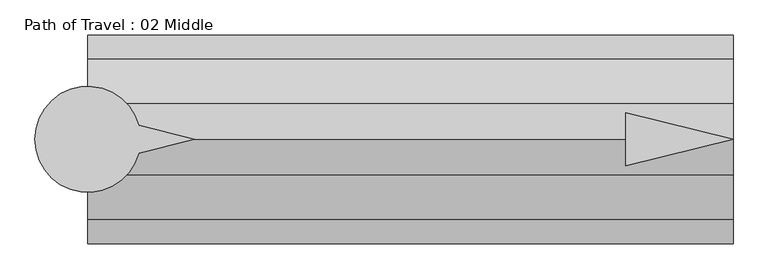
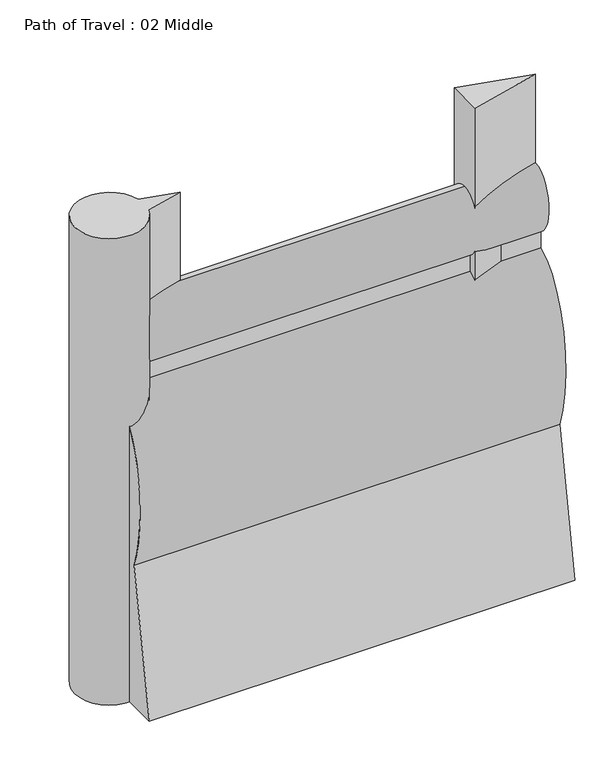
"""IFC4 building model written with IfcOpenShell, lengths in millimetres: proxy geometry, Path of Travel : 02 Middle."""

from ifc_helpers import new_model, si_unit, point, frame, frame_2d, origin, origin_with_axes, place, context, project, spatial, polyline, circle_curve, ellipse_curve, trimmed, segment, composite_curve, outline, extrude, source, transform, mapped, element, save
from ifc_brep_helpers import plane_surface, extruded_surface, advanced_brep


def path_of_travel_02_middle_c901b5b9(model_context):
    return source(origin(), model_context, "Body", "SolidModel", [
        advanced_brep(
        [(227.5554837, 0.0, 1727.2), (227.5554837, 42.9018657, 1436.6534209), (227.5554837, 42.9018657, 1363.4763406), (227.5554837, 184.1186263, 643.4144547), (227.5554837, 297.5699544, 0.0), (227.5554837, 145.6574193, 0.0), (227.5554837, 0.0, 584.2), (227.5554837, -145.6574193, 0.0), (227.5554837, -297.5699544, 0.0), (227.5554837, -184.1186263, 643.4144547), (227.5554837, -42.9018657, 1363.4763406), (227.5554837, -42.9018657, 1436.6534209), (2067.1704554, 0.0, 1727.2), (2067.1704554, -42.9018657, 1436.6534209), (2067.1704554, -42.9018657, 1363.4763406), (2067.1704554, -184.1186263, 643.4144547), (2067.1704554, -297.5699544, 0.0), (2067.1704554, -145.6574193, 0.0), (2067.1704554, 0.0, 584.2), (2067.1704554, 145.6574193, 0.0), (2067.1704554, 297.5699544, 0.0), (2067.1704554, 184.1186263, 643.4144547), (2067.1704554, 42.9018657, 1363.4763406), (2067.1704554, 42.9018657, 1436.6534209)],
        [
            (0, 1, ellipse_curve(frame((227.5554837, 0.0, 1574.8), z_axis=(-1.0, 0.0, 0.0), x_axis=(0.0, 0.0, 1.0)), 152.4, 101.6)),
            (1, 2),
            (2, 3, ellipse_curve(frame((227.5554837, 0.0, 914.4), z_axis=(-1.0, 0.0, 0.0), x_axis=(0.0, 0.0, -1.0)), 457.2, 228.6)),
            (3, 4),
            (4, 5),
            (5, 6),
            (6, 7),
            (7, 8),
            (8, 9),
            (9, 10, ellipse_curve(frame((227.5554837, 0.0, 914.4), z_axis=(-1.0, 0.0, 0.0), x_axis=(0.0, 0.0, -1.0)), 457.2, 228.6)),
            (10, 11),
            (11, 0, ellipse_curve(frame((227.5554837, 0.0, 1574.8), z_axis=(-1.0, 0.0, 0.0), x_axis=(0.0, 0.0, 1.0)), 152.4, 101.6)),
            (12, 13, ellipse_curve(frame((2067.1704554, 0.0, 1574.8), z_axis=(1.0, 0.0, 0.0), x_axis=(0.0, 0.0, 1.0)), 152.4, 101.6)),
            (13, 14),
            (14, 15, ellipse_curve(frame((2067.1704554, 0.0, 914.4), z_axis=(1.0, 0.0, 0.0), x_axis=(0.0, 0.0, -1.0)), 457.2, 228.6)),
            (15, 16),
            (16, 17),
            (17, 18),
            (18, 19),
            (19, 20),
            (20, 21),
            (21, 22, ellipse_curve(frame((2067.1704554, 0.0, 914.4), z_axis=(1.0, 0.0, 0.0), x_axis=(0.0, 0.0, -1.0)), 457.2, 228.6)),
            (22, 23),
            (23, 12, ellipse_curve(frame((2067.1704554, 0.0, 1574.8), z_axis=(1.0, 0.0, 0.0), x_axis=(0.0, 0.0, 1.0)), 152.4, 101.6)),
            (0, 12),
            (23, 1),
            (22, 2),
            (21, 3),
            (20, 4),
            (19, 5),
            (18, 6),
            (17, 7),
            (16, 8),
            (15, 9),
            (14, 10),
            (13, 11),
        ],
        [
            plane_surface(frame((227.5554837, 0.0, 0.0), z_axis=(-1.0, 0.0, 0.0), x_axis=(0.0, 0.0, 1.0))),
            plane_surface(frame((2067.1704554, 0.0, 0.0), z_axis=(1.0, 0.0, 0.0), x_axis=(0.0, 0.0, 1.0))),
            extruded_surface(trimmed(ellipse_curve(frame((2067.1704554, 0.0, 1574.8), z_axis=(-1.0, 0.0, 0.0), x_axis=(0.0, 0.0, 1.0)), 152.4, 101.6), [point((2067.1704554, 0.0, 1727.2))], [point((2067.1704554, 42.9018657, 1436.6534209))], True, "CARTESIAN"), (-1839.6149716999998, 0.0, 0.0), 1839.6149716999998),
            plane_surface(frame((227.5554837, 42.9018657, 1436.6534209), z_axis=(0.0, 1.0, 0.0), x_axis=(1.0, 0.0, 0.0))),
            extruded_surface(trimmed(ellipse_curve(frame((2067.1704554, 0.0, 914.4), z_axis=(-1.0, 0.0, 0.0), x_axis=(0.0, 0.0, -1.0)), 457.2, 228.6), [point((2067.1704554, 42.9018657, 1363.4763406))], [point((2067.1704554, 184.1186263, 643.4144547))], True, "CARTESIAN"), (-1839.6149716999998, 0.0, 0.0), 1839.6149716999998),
            plane_surface(frame((227.5554837, 184.1186263, 643.4144547), z_axis=(0.0, 0.9848077530122078, 0.1736481776669322), x_axis=(1.0, 0.0, 0.0))),
            plane_surface(frame((227.5554837, 297.5699544, 0.0), z_axis=(0.0, 0.0, -1.0), x_axis=(1.0, 0.0, 0.0))),
            plane_surface(frame((227.5554837, 145.6574193, 0.0), z_axis=(0.0, -0.9702957262760199, -0.2419218955995739), x_axis=(1.0, 0.0, 0.0))),
            plane_surface(frame((227.5554837, 0.0, 584.2), z_axis=(0.0, 0.9702957262759961, -0.24192189559966923), x_axis=(1.0, 0.0, 0.0))),
            plane_surface(frame((227.5554837, -145.6574193, 0.0), z_axis=(0.0, 0.0, -1.0), x_axis=(1.0, 0.0, 0.0))),
            plane_surface(frame((227.5554837, -297.5699544, 0.0), z_axis=(0.0, -0.984807753012208, 0.17364817766693066), x_axis=(1.0, 0.0, 0.0))),
            extruded_surface(trimmed(ellipse_curve(frame((2067.1704554, 0.0, 914.4), z_axis=(-1.0, 0.0, 0.0), x_axis=(0.0, 0.0, -1.0)), 457.2, 228.6), [point((2067.1704554, -184.1186263, 643.4144547))], [point((2067.1704554, -42.9018657, 1363.4763406))], True, "CARTESIAN"), (-1839.6149716999998, 0.0, 0.0), 1839.6149716999998),
            plane_surface(frame((227.5554837, -42.9018657, 1363.4763406), z_axis=(0.0, -1.0, 0.0), x_axis=(1.0, 0.0, 0.0))),
            extruded_surface(trimmed(ellipse_curve(frame((2067.1704554, 0.0, 1574.8), z_axis=(-1.0, 0.0, 0.0), x_axis=(0.0, 0.0, 1.0)), 152.4, 101.6), [point((2067.1704554, -42.9018657, 1436.6534209))], [point((2067.1704554, 0.0, 1727.2))], True, "CARTESIAN"), (-1839.6149716999998, 0.0, 0.0), 1839.6149716999998),
        ],
        [
            (0, [[1, 2, 3, 4, 5, 6, 7, 8, 9, 10, 11, 12]]),
            (1, [[13, 14, 15, 16, 17, 18, 19, 20, 21, 22, 23, 24]]),
            (2, [[-1, 25, -24, 26]]),
            (3, [[-2, -26, -23, 27]]),
            (4, [[-3, -27, -22, 28]]),
            (5, [[-4, -28, -21, 29]]),
            (6, [[-5, -29, -20, 30]]),
            (7, [[-6, -30, -19, 31]]),
            (8, [[-7, -31, -18, 32]]),
            (9, [[-8, -32, -17, 33]]),
            (10, [[-9, -33, -16, 34]]),
            (11, [[-10, -34, -15, 35]]),
            (12, [[-11, -35, -14, 36]]),
            (13, [[-12, -36, -13, -25]]),
        ],
    ),
        extrude(outline(polyline([(1761.1653088, 76.2006338), (2067.1704554, 0.0), (1761.1653088, -76.2006338), (1761.1653088, 76.2006338)])), origin_with_axes(), (0.0, 0.0, 1.0), 2129.5973753),
        extrude(outline(composite_curve([segment(polyline([(372.7837828, 39.4440225), (531.182385, 0.0), (372.7837828, -39.4440225)]), True, "CONTINUOUS"), segment(trimmed(circle_curve(frame_2d((227.2200886, 0.0)), 150.8131956), [point((372.7837828, -39.4440225))], [point((372.7837828, 39.4440225))], False, "CARTESIAN"), True, "CONTINUOUS")], self_intersect=False)), origin_with_axes(), (0.0, 0.0, 1.0), 2129.5973753),
    ])


if __name__ == "__main__":
    model = new_model("IFC4")
    model_context = context("Model", 3, world=origin())
    ifc_project = project(units=[si_unit("LENGTHUNIT", "METRE", prefix="MILLI")], contexts=[model_context])
    site = spatial("IfcSite", under=ifc_project)
    building = spatial("IfcBuilding", under=site)
    placement = place(None, origin())
    path_of_travel_02_middle_shape = path_of_travel_02_middle_c901b5b9(model_context)
    element("IfcBuildingElementProxy", 1, Name="Path of Travel : 02 Middle", ObjectType="Path of Travel : 02 Middle", at=placement, inside=building, context=model_context, shape_type="MappedRepresentation", body=[
        mapped(path_of_travel_02_middle_shape, transform((0.0, 0.0, 0.0), x_axis=(1.0, 0.0, 0.0), y_axis=(0.0, 1.0, 0.0), z_axis=(0.0, 0.0, 1.0))),
    ])
    save(model, "model.ifc")

# Revit data of these elements
# Type "Path of Travel : 02 Middle"
#   Path of Egress [instance default] = 4' - 0"
#   built-in parameter 1001306 [instance default] = 4 (stored number, unit not read)
#   Dot at Start = no
#   Arrow in Middle = yes
#   Arrow at End = no
#   Egress Path = none
# Element 1 (IfcBuildingElementProxy, "Path of Travel : 02 Middle")
#   Path of Egress = 6' - 0 109/256"
#   built-in parameter 1001306 = 6.03548 (stored number, unit not read)
#   Materials on its faces: "Egress Path Solid", "solid"
# Materials
#   "Egress Path Solid": class "Unassigned", colour RGB 255 128 64, transparency 0.75, Comments = "Rendering appearance not upgraded "
#   "solid": class "Generic", colour RGB 120 120 120, transparency 0, Cost = 0
